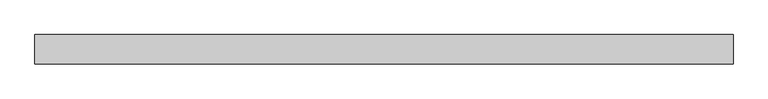
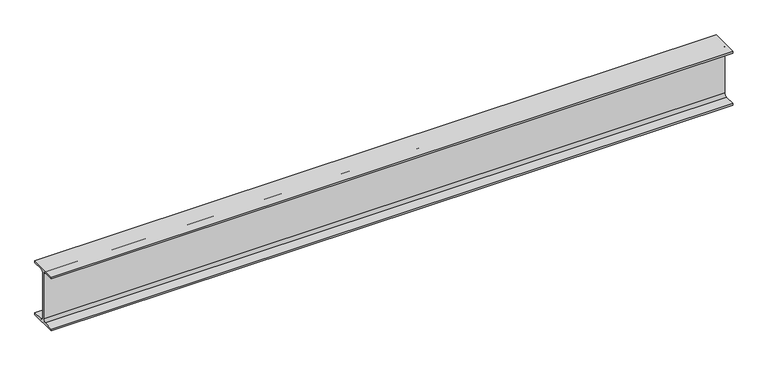
"""IFC4 building model written with IfcOpenShell, lengths in millimetres: beam geometry, 0912_Steel Framing_H-KSD3502 : H_SB_ASB_H-250x125x6x9."""

from ifc_helpers import new_model, si_unit, point, frame, frame_2d, origin, place, context, project, spatial, polyline, circle_curve, trimmed, segment, composite_curve, outline, extrude, source, transform, mapped, element, save


def beam_64758b51(model_context):
    return source(origin(), model_context, "Body", "SweptSolid", [
        extrude(outline(composite_curve([segment(polyline([(62.5, -116.0), (62.5, -125.0), (-62.5, -125.0), (-62.5, -116.0), (-15.0, -116.0)]), True, "CONTINUOUS"), segment(trimmed(circle_curve(frame_2d((-15.0, -104.0)), 12.0), [point((-15.0, -116.0))], [point((-3.0, -104.0))], True, "CARTESIAN"), True, "CONTINUOUS"), segment(polyline([(-3.0, -104.0), (-3.0, 104.0)]), True, "CONTINUOUS"), segment(trimmed(circle_curve(frame_2d((-15.0, 104.0)), 12.0), [point((-3.0, 104.0))], [point((-15.0, 116.0))], True, "CARTESIAN"), True, "CONTINUOUS"), segment(polyline([(-15.0, 116.0), (-62.5, 116.0), (-62.5, 125.0), (62.5, 125.0), (62.5, 116.0), (15.0, 116.0)]), True, "CONTINUOUS"), segment(trimmed(circle_curve(frame_2d((15.0, 104.0)), 12.0), [point((15.0, 116.0))], [point((3.0, 104.0))], True, "CARTESIAN"), True, "CONTINUOUS"), segment(polyline([(3.0, 104.0), (3.0, -104.0)]), True, "CONTINUOUS"), segment(trimmed(circle_curve(frame_2d((15.0, -104.0)), 12.0), [point((3.0, -104.0))], [point((15.0, -116.0))], True, "CARTESIAN"), True, "CONTINUOUS"), segment(polyline([(15.0, -116.0), (62.5, -116.0)]), True, "CONTINUOUS")], self_intersect=False)), frame((-1493.3, 0.0, 0.0), z_axis=(1.0, 0.0, 0.0), x_axis=(0.0, 1.0, 0.0)), (0.0, 0.0, 1.0), 2987.8360727),
    ])


if __name__ == "__main__":
    model = new_model("IFC4")
    model_context = context("Model", 3, world=origin())
    ifc_project = project(units=[si_unit("LENGTHUNIT", "METRE", prefix="MILLI")], contexts=[model_context])
    site = spatial("IfcSite", under=ifc_project)
    building = spatial("IfcBuilding", under=site)
    placement = place(None, origin())
    beam_shape = beam_64758b51(model_context)
    element("IfcBeam", 1, ObjectType="0912_Steel Framing_H-KSD3502 : H_SB_ASB_H-250x125x6x9", at=placement, inside=building, context=model_context, shape_type="MappedRepresentation", body=[
        mapped(beam_shape, transform((0.0, 0.0, 0.0), x_axis=(1.0, 0.0, 0.0), y_axis=(0.0, 1.0, 0.0), z_axis=(0.0, 0.0, 1.0))),
    ])
    save(model, "model.ifc")

# Revit data of these elements
# Type "0912_Steel Framing_H-KSD3502 : H_SB_ASB_H-250x125x6x9"
#   H_WM Code_1 = "S01AA003-00001 | Main Steel Structure Fabrication Work | Shelter/Building | Light Steel - Standard (30KG/M>Weight) | Material: (   )"
#   H_WM Code_2 = "S03AA029-00001 | Main Steel Structure Erection Work | Shelter/Building | Light Steel (30KG/M>Weight) | Material: (   )"
#   H_WM Code_3 = "S01AA010-00001 | Main Steel Structure Fabrication Work | Shelter/Building | Steel Painting/Coating | for Non-Fireproofed Steel Surface, Surface Preparation, Primer, Second & Final Coat | Material: (   )"
#   H_Q'ty Cal Type Tag = "SB-Q2"
#   Width = 12.5 cm
#   Web Thickness = 0.6 cm
#   Web Fillet = 1.2 cm
#   Warping Constant = 42539.8 cm⁶
#   W = 0
#   Torsional Moment of Inertia = 7.8102 cm⁴
#   Section Area = 37.66 cm²
#   Plastic Modulus weak axis = 73.1 cm³
#   Plastic Modulus strong axis = 366.0 cm³
#   Perimeter = 0.97 m²/m
#   Nominal Weight = 29.60 kgf/m
#   Moment of Inertia weak axis = 294.00 cm⁴
#   Moment of Inertia strong axis = 4050.00 cm⁴
#   Height = 25.0 cm
#   Flange Thickness = 0.9 cm
#   Elastic Modulus weak axis = 47.0 cm³
#   Elastic Modulus strong axis = 324.0 cm³
#   Centroid Vertical = 12.5 cm
#   Centroid Horizontal = 6.25 cm
#   Ix = 40500000
#   Length [instance default] = 1.5240 m
#   Zx = 366000
#   b = 0.1250 m
#   h = 0.2500 m
#   r = 0.0120 m
#   s = 0.0060 m
#   t = 0.0090 m
#   A = 0.003766 m²
#   Structural Material [instance default] = Steel, 45-345
#   Assembly Code = ""
# Element 1 (IfcBeam, "0912_Steel Framing_H-KSD3502 : H_SB_ASB_H-250x125x6x9")
#   Structural Material = none
# Materials
#   "Steel, 45-345": class "Metal", colour RGB 189 187 185, transparency 0, Description = "Steel 345 MPa", Cost = 0
